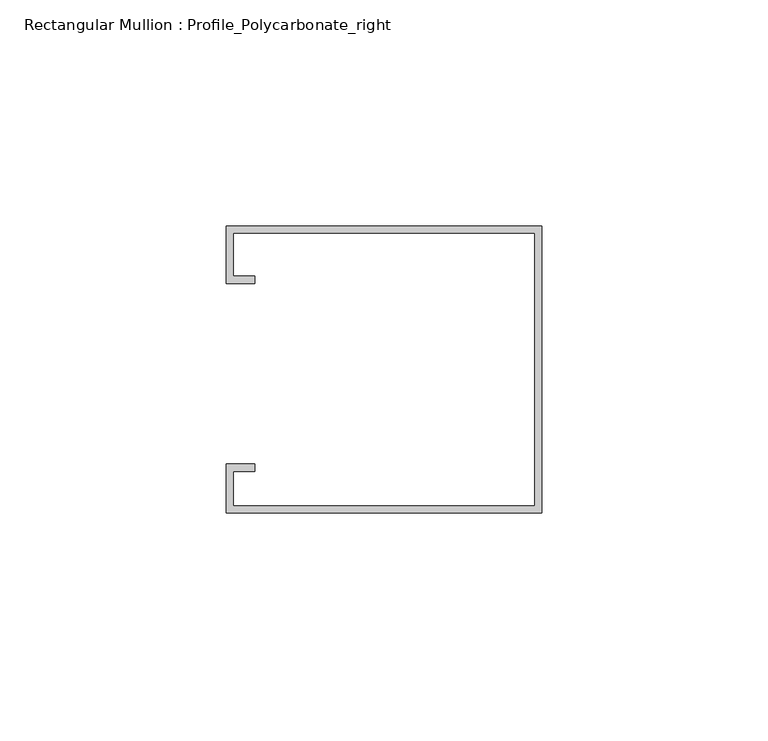
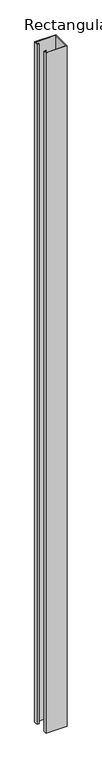
"""IFC4 building model written with IfcOpenShell, lengths in millimetres: member geometry, Rectangular Mullion : Profile_Polycarbonate_right."""

from ifc_helpers import new_model, si_unit, frame, origin, place, context, project, spatial, polyline, outline, extrude, source, transform, mapped, element, save


def rectangular_mullion_profile_polycarbonate_right_1eff4e41(model_context):
    return source(origin(), model_context, "Body", "SweptSolid", [
        extrude(outline(polyline([(0.0, 32.7), (0.0, -30.8), (-69.85, -30.8), (-69.85, -20.0), (-63.5, -20.0), (-63.5, -21.5875), (-68.2625, -21.5875), (-68.2625, -29.2125), (-1.5875, -29.2125), (-1.5875, 31.1125), (-68.2625, 31.1125), (-68.2625, 21.5875), (-63.5, 21.5875), (-63.5, 20.0), (-69.85, 20.0), (-69.85, 32.7), (0.0, 32.7)])), frame((0.0, 0.0, -2369.6313366), z_axis=(0.0, 0.0, 1.0), x_axis=(1.0, 0.0, 0.0)), (0.0, 0.0, 1.0), 2369.6313366),
    ])


if __name__ == "__main__":
    model = new_model("IFC4")
    model_context = context("Model", 3, world=origin())
    ifc_project = project(units=[si_unit("LENGTHUNIT", "METRE", prefix="MILLI")], contexts=[model_context])
    site = spatial("IfcSite", under=ifc_project)
    building = spatial("IfcBuilding", under=site)
    placement = place(None, origin())
    rectangular_mullion_profile_polycarbonate_right_shape = rectangular_mullion_profile_polycarbonate_right_1eff4e41(model_context)
    element("IfcMember", 1, ObjectType="Rectangular Mullion : Profile_Polycarbonate_right", at=placement, inside=building, context=model_context, shape_type="MappedRepresentation", body=[
        mapped(rectangular_mullion_profile_polycarbonate_right_shape, transform((0.0, 0.0, 0.0), x_axis=(1.0, 0.0, 0.0), y_axis=(0.0, 1.0, 0.0), z_axis=(0.0, 0.0, 1.0))),
    ])
    save(model, "model.ifc")

# Revit data of these elements
# Type "Rectangular Mullion : Profile_Polycarbonate_right"
#   built-in parameter 1007322 = 0.208333 (stored number, unit not read)
#   built-in parameter 1007321 = 0 (stored number, unit not read)
#   built-in parameter 1007320 = 0.00520833 (stored number, unit not read)
